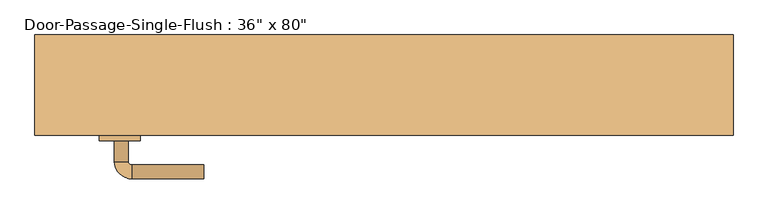
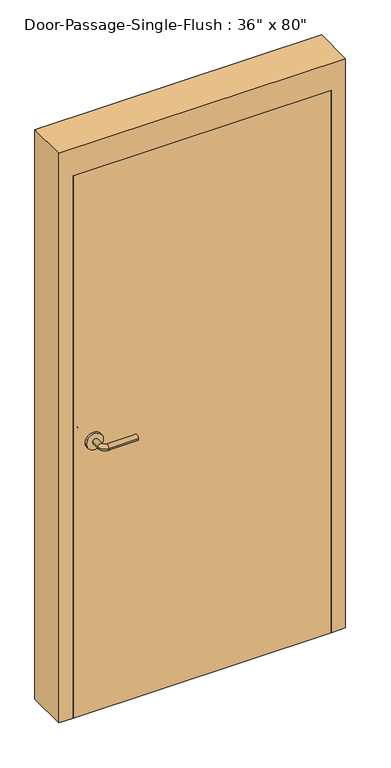
"""IFC4 building model written with IfcOpenShell, lengths in millimetres: door geometry."""

from ifc_helpers import new_model, si_unit, point, frame, frame_2d, origin, origin_with_axes, place, context, project, spatial, polyline, circle_curve, ellipse_curve, trimmed, segment, composite_curve, outline, extrude, faceted_brep, source, transform, mapped, element, save
from ifc_brep_helpers import plane_surface, cylinder_surface, revolved_surface, advanced_brep


def door_15b50305(model_context):
    return source(origin(), model_context, "Body", "SolidModel", [
        advanced_brep(
        [(-392.190625, -26.925, 1016.0), (-372.190625, -26.925, 1016.0), (-392.190625, 3.075, 1016.0), (-372.190625, 3.075, 1016.0), (-367.190625, 8.075, 1016.0), (-367.190625, 28.075, 1016.0), (-262.190625, 28.075, 1016.0), (-262.190625, 8.075, 1016.0)],
        [
            (0, 1, circle_curve(frame((-382.190625, -26.925, 1016.0), z_axis=(0.0, -1.0, 0.0), x_axis=(1.0, 0.0, 0.0)), 10.0)),
            (1, 0, circle_curve(frame((-382.190625, -26.925, 1016.0), z_axis=(0.0, -1.0, 0.0), x_axis=(1.0, 0.0, 0.0)), 10.0)),
            (0, 2),
            (2, 3, circle_curve(frame((-382.190625, 3.075, 1016.0), z_axis=(0.0, -1.0, 0.0), x_axis=(1.0, 0.0, 0.0)), 10.0)),
            (3, 1),
            (3, 2, circle_curve(frame((-382.190625, 3.075, 1016.0), z_axis=(0.0, -1.0, 0.0), x_axis=(1.0, 0.0, 0.0)), 10.0)),
            (4, 3, circle_curve(frame((-367.190625, 3.075, 1016.0), z_axis=(0.0, 0.0, 1.0), x_axis=(-1.0, 0.0, 0.0)), 5.0)),
            (2, 5, circle_curve(frame((-367.190625, 3.075, 1016.0), z_axis=(0.0, 0.0, -1.0), x_axis=(-1.0, 0.0, 0.0)), 25.0)),
            (5, 4, circle_curve(frame((-367.190625, 18.075, 1016.0), z_axis=(-1.0, 0.0, 0.0), x_axis=(0.0, -1.0, 0.0)), 10.0)),
            (4, 5, circle_curve(frame((-367.190625, 18.075, 1016.0), z_axis=(-1.0, 0.0, 0.0), x_axis=(0.0, -1.0, 0.0)), 10.0)),
            (6, 7, circle_curve(frame((-262.190625, 18.075, 1016.0), z_axis=(1.0, 0.0, 0.0), x_axis=(0.0, -1.0, 0.0)), 10.0)),
            (7, 6, circle_curve(frame((-262.190625, 18.075, 1016.0), z_axis=(1.0, 0.0, 0.0), x_axis=(0.0, -1.0, 0.0)), 10.0)),
            (5, 6),
            (7, 4),
        ],
        [
            plane_surface(frame((-382.190625, -26.925, 1016.0), z_axis=(0.0, -1.0, 0.0), x_axis=(0.0, 0.0, 1.0))),
            cylinder_surface(frame((-382.190625, -26.925, 1016.0), z_axis=(0.0, -1.0, 0.0), x_axis=(1.0, 0.0, 0.0)), 10.0),
            revolved_surface(trimmed(ellipse_curve(frame((-382.190625, 3.075, 1016.0), z_axis=(0.0, -1.0, 0.0), x_axis=(1.0, 0.0, 0.0)), 10.0, 10.0), [point((-392.190625, 3.075, 1016.0))], [point((-372.190625, 3.075, 1016.0))], True, "CARTESIAN"), (-367.190625, 3.075, 1016.0), (0.0, 0.0, -1.0)),
            revolved_surface(trimmed(ellipse_curve(frame((-382.190625, 3.075, 1016.0), z_axis=(0.0, -1.0, 0.0), x_axis=(1.0, 0.0, 0.0)), 10.0, 10.0), [point((-372.190625, 3.075, 1016.0))], [point((-392.190625, 3.075, 1016.0))], True, "CARTESIAN"), (-367.190625, 3.075, 1016.0), (0.0, 0.0, -1.0)),
            plane_surface(frame((-262.190625, 18.075, 1016.0), z_axis=(1.0, 0.0, 0.0), x_axis=(0.0, 0.0, 1.0))),
            cylinder_surface(frame((-367.190625, 18.075, 1016.0), z_axis=(-1.0, 0.0, 0.0), x_axis=(0.0, -1.0, 0.0)), 10.0),
        ],
        [
            (0, [[1, 2]]),
            (1, [[-1, 3, 4, 5]]),
            (1, [[-2, -5, 6, -3]]),
            (2, [[7, -4, 8, 9]]),
            (3, [[-8, -6, -7, 10]]),
            (4, [[11, 12]]),
            (5, [[-9, 13, -12, 14]]),
            (5, [[-10, -14, -11, -13]]),
        ],
    ),
        extrude(outline(composite_curve([segment(trimmed(circle_curve(frame_2d((1016.0, -384.690625)), 30.0), [point((1016.0, -414.690625))], [point((1016.0, -354.690625))], False, "CARTESIAN"), True, "CONTINUOUS"), segment(trimmed(circle_curve(frame_2d((1016.0, -384.690625)), 30.0), [point((1016.0, -354.690625))], [point((1016.0, -414.690625))], False, "CARTESIAN"), True, "CONTINUOUS")], self_intersect=False)), frame((0.0, -34.925, 0.0), z_axis=(0.0, 1.0, 0.0), x_axis=(0.0, 0.0, 1.0)), (0.0, 0.0, 1.0), 8.0),
        advanced_brep(
        [(-392.190625, -87.375, 1016.0), (-372.190625, -87.375, 1016.0), (-372.190625, -117.375, 1016.0), (-392.190625, -117.375, 1016.0), (-367.190625, -122.375, 1016.0), (-367.190625, -142.375, 1016.0), (-262.190625, -142.375, 1016.0), (-262.190625, -122.375, 1016.0)],
        [
            (0, 1, circle_curve(frame((-382.190625, -87.375, 1016.0), z_axis=(0.0, 1.0, 0.0), x_axis=(1.0, 0.0, 0.0)), 10.0)),
            (1, 0, circle_curve(frame((-382.190625, -87.375, 1016.0), z_axis=(0.0, 1.0, 0.0), x_axis=(1.0, 0.0, 0.0)), 10.0)),
            (1, 2),
            (2, 3, circle_curve(frame((-382.190625, -117.375, 1016.0), z_axis=(0.0, 1.0, 0.0), x_axis=(1.0, 0.0, 0.0)), 10.0)),
            (3, 0),
            (3, 2, circle_curve(frame((-382.190625, -117.375, 1016.0), z_axis=(0.0, 1.0, 0.0), x_axis=(1.0, 0.0, 0.0)), 10.0)),
            (4, 5, circle_curve(frame((-367.190625, -132.375, 1016.0), z_axis=(-1.0, 0.0, 0.0), x_axis=(0.0, 1.0, 0.0)), 10.0)),
            (5, 3, circle_curve(frame((-367.190625, -117.375, 1016.0), z_axis=(0.0, 0.0, -1.0), x_axis=(-1.0, 0.0, 0.0)), 25.0)),
            (2, 4, circle_curve(frame((-367.190625, -117.375, 1016.0), z_axis=(0.0, 0.0, 1.0), x_axis=(-1.0, 0.0, 0.0)), 5.0)),
            (5, 4, circle_curve(frame((-367.190625, -132.375, 1016.0), z_axis=(-1.0, 0.0, 0.0), x_axis=(0.0, 1.0, 0.0)), 10.0)),
            (6, 7, circle_curve(frame((-262.190625, -132.375, 1016.0), z_axis=(1.0, 0.0, 0.0), x_axis=(0.0, 1.0, 0.0)), 10.0)),
            (7, 6, circle_curve(frame((-262.190625, -132.375, 1016.0), z_axis=(1.0, 0.0, 0.0), x_axis=(0.0, 1.0, 0.0)), 10.0)),
            (4, 7),
            (6, 5),
        ],
        [
            plane_surface(frame((-382.190625, -87.375, 1016.0), z_axis=(0.0, 1.0, 0.0), x_axis=(0.0, 0.0, 1.0))),
            cylinder_surface(frame((-382.190625, -87.375, 1016.0), z_axis=(0.0, 1.0, 0.0), x_axis=(1.0, 0.0, 0.0)), 10.0),
            revolved_surface(trimmed(ellipse_curve(frame((-382.190625, -117.375, 1016.0), z_axis=(0.0, -1.0, 0.0), x_axis=(1.0, 0.0, 0.0)), 10.0, 10.0), [point((-392.190625, -117.375, 1016.0))], [point((-372.190625, -117.375, 1016.0))], True, "CARTESIAN"), (-367.190625, -117.375, 1016.0), (0.0, 0.0, -1.0)),
            revolved_surface(trimmed(ellipse_curve(frame((-382.190625, -117.375, 1016.0), z_axis=(0.0, -1.0, 0.0), x_axis=(1.0, 0.0, 0.0)), 10.0, 10.0), [point((-372.190625, -117.375, 1016.0))], [point((-392.190625, -117.375, 1016.0))], True, "CARTESIAN"), (-367.190625, -117.375, 1016.0), (0.0, 0.0, -1.0)),
            plane_surface(frame((-262.190625, -132.375, 1016.0), z_axis=(1.0, 0.0, 0.0), x_axis=(0.0, 0.0, 1.0))),
            cylinder_surface(frame((-367.190625, -132.375, 1016.0), z_axis=(-1.0, 0.0, 0.0), x_axis=(0.0, 1.0, 0.0)), 10.0),
        ],
        [
            (0, [[1, 2]]),
            (1, [[3, 4, 5, -2]]),
            (1, [[-5, 6, -3, -1]]),
            (2, [[7, 8, -4, 9]]),
            (3, [[10, -9, -6, -8]]),
            (4, [[11, 12]]),
            (5, [[13, -11, 14, -7]]),
            (5, [[-14, -12, -13, -10]]),
        ],
    ),
        extrude(outline(composite_curve([segment(trimmed(circle_curve(frame_2d((1016.0, -384.690625)), 30.0), [point((1016.0, -414.690625))], [point((1016.0, -354.690625))], False, "CARTESIAN"), True, "CONTINUOUS"), segment(trimmed(circle_curve(frame_2d((1016.0, -384.690625)), 30.0), [point((1016.0, -354.690625))], [point((1016.0, -414.690625))], False, "CARTESIAN"), True, "CONTINUOUS")], self_intersect=False)), frame((0.0, -87.375, 0.0), z_axis=(0.0, 1.0, 0.0), x_axis=(0.0, 0.0, 1.0)), (0.0, 0.0, 1.0), 8.0),
        faceted_brep([(457.2, -30.1625, 0.0), (441.325, -30.1625, 0.0), (441.325, 17.4625, 0.0), (457.2, 17.4625, 0.0), (457.2, 66.675, 0.0), (508.0, 66.675, 0.0), (508.0, -79.375, 0.0), (457.2, -79.375, 0.0), (457.2, -79.375, 2032.0), (457.2, -30.1625, 2032.0), (508.0, -79.375, 2133.6), (-508.0, -79.375, 2133.6), (-508.0, -79.375, 0.0), (-457.2, -79.375, 0.0), (-457.2, -79.375, 2032.0), (508.0, 66.675, 2133.6), (457.2, 66.675, 2032.0), (-457.2, 66.675, 2032.0), (-457.2, 66.675, 0.0), (-508.0, 66.675, 0.0), (-508.0, 66.675, 2133.6), (457.2, 17.4625, 2032.0), (441.325, 17.4625, 2016.125), (-441.325, 17.4625, 2016.125), (-441.325, 17.4625, 0.0), (-457.2, 17.4625, 0.0), (-457.2, 17.4625, 2032.0), (441.325, -30.1625, 2016.125), (-457.2, -30.1625, 2032.0), (-457.2, -30.1625, 0.0), (-441.325, -30.1625, 0.0), (-441.325, -30.1625, 2016.125)], [[[0, 1, 2, 3, 4, 5, 6, 7]], [[7, 8, 9, 0]], [[6, 10, 11, 12, 13, 14, 8, 7]], [[5, 15, 10, 6]], [[4, 16, 17, 18, 19, 20, 15, 5]], [[3, 21, 16, 4]], [[2, 22, 23, 24, 25, 26, 21, 3]], [[1, 27, 22, 2]], [[0, 9, 28, 29, 30, 31, 27, 1]], [[8, 14, 28, 9]], [[16, 21, 26, 17]], [[22, 27, 31, 23]], [[12, 19, 18, 25, 24, 30, 29, 13]], [[13, 29, 28, 14]], [[11, 20, 19, 12]], [[17, 26, 25, 18]], [[23, 31, 30, 24]], [[15, 20, 11, 10]]]),
        extrude(outline(polyline([(457.2, -34.925), (457.2, -79.375), (-457.2, -79.375), (-457.2, -34.925), (457.2, -34.925)])), origin_with_axes(), (0.0, 0.0, 1.0), 2032.0),
    ])


if __name__ == "__main__":
    model = new_model("IFC4")
    model_context = context("Model", 3, world=origin())
    ifc_project = project(units=[si_unit("LENGTHUNIT", "METRE", prefix="MILLI")], contexts=[model_context])
    site = spatial("IfcSite", under=ifc_project)
    building = spatial("IfcBuilding", under=site)
    placement = place(None, origin())
    door_shape = door_15b50305(model_context)
    element("IfcDoor", 1, ObjectType="Door-Passage-Single-Flush : 36\" x 80\"", at=placement, inside=building, context=model_context, shape_type="MappedRepresentation", body=[
        mapped(door_shape, transform((0.0, 0.0, 0.0), x_axis=(1.0, 0.0, 0.0), y_axis=(0.0, 1.0, 0.0), z_axis=(0.0, 0.0, 1.0))),
    ])
    save(model, "model.ifc")

# Revit data of these elements
# Type "Door-Passage-Single-Flush : 36\" x 80\""
#   Type Mark = "16"
#   Assembly Code = "B2030200"
#   Analytic Construction = "Wooden"
#   Thickness = 0' - 1 3/4"
#   Thermal Resistance (R) = 0.455703 (m²·K)/W
#   Swing Angle [instance default] = 90.00°
#   Strike Height = 3' - 4"
#   Rough Width [instance default] = 3' - 4"
#   Rough Height [instance default] = 7' - 0"
#   MF Opening Height [instance default] = 0' - 4"
#   MF Opening Width [instance default] = 0' - 4"
#   Inset Calculate [instance default] = 0' - 4"
#   Masonry Inset [instance default] = 0' - 1"
#   Height = 6' - 8"
#   Width = 3' - 0"
#   Heat Transfer Coefficient (U) = 2.19465 W/(m²·K)
#   Masonry Frame Depth = 0' - 5 3/4"
#   Masonry Frame [instance default] = yes
#   Function = 1
#   Dry Wall Frame [instance default] = no
#   Panel Material = Wood - Birch
#   Frame Material = Metal - Paint Finish - Grey
#   Door Handle Material = Aluminum
#   Visual Light Transmittance = 0
#   Solar Heat Gain Coefficient = 0
#   Wall Closure = (empty or 0)
# Element 1 (IfcDoor, "Door-Passage-Single-Flush : 36\" x 80\"")
#   Inset Calculate = 0' - 2 1/2"
#   Masonry Inset = -0' - 0 1/2"
#   Materials on its faces: "Aluminum", "Metal - Paint Finish - Grey", "Wood - Birch"
# Materials
#   "Wood - Birch": class "Wood", colour RGB 166 116 52, transparency 0, Cost = 0
#   "Metal - Paint Finish - Grey": class "Paint", colour RGB 104 104 104, transparency 0, Cost = 0
#   "Aluminum": class "Metal", colour RGB 247 247 247, transparency 0, Description = "Aluminum 6061", Cost = 0
